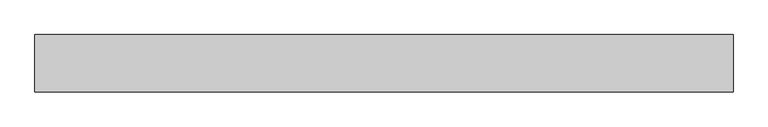
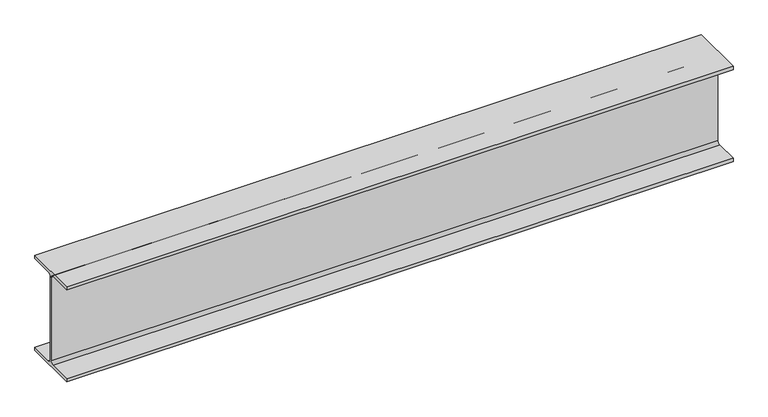
"""IFC4 building model written with IfcOpenShell, lengths in millimetres: beam geometry, Old_Steel Beam_H-KSD3502 : H_SB_ASB_H-194×150x6x9."""

from ifc_helpers import new_model, si_unit, point, frame, frame_2d, origin, place, context, project, spatial, polyline, circle_curve, trimmed, segment, composite_curve, outline, extrude, source, transform, mapped, element, save


def beam_e603d65a(model_context):
    return source(origin(), model_context, "Body", "SweptSolid", [
        extrude(outline(composite_curve([segment(polyline([(-82.5, -141.5), (-11.9, -141.5)]), True, "CONTINUOUS"), segment(trimmed(circle_curve(frame_2d((-11.9, -132.6)), 8.9), [point((-11.9, -141.5))], [point((-3.0, -132.6))], True, "CARTESIAN"), True, "CONTINUOUS"), segment(polyline([(-3.0, -132.6), (-3.0, 132.6)]), True, "CONTINUOUS"), segment(trimmed(circle_curve(frame_2d((-11.9, 132.6)), 8.9), [point((-3.0, 132.6))], [point((-11.9, 141.5))], True, "CARTESIAN"), True, "CONTINUOUS"), segment(polyline([(-11.9, 141.5), (-82.5, 141.5), (-82.5, 151.7), (82.5, 151.7), (82.5, 141.5), (11.9, 141.5)]), True, "CONTINUOUS"), segment(trimmed(circle_curve(frame_2d((11.9, 132.6)), 8.9), [point((11.9, 141.5))], [point((3.0, 132.6))], True, "CARTESIAN"), True, "CONTINUOUS"), segment(polyline([(3.0, 132.6), (3.0, -132.6)]), True, "CONTINUOUS"), segment(trimmed(circle_curve(frame_2d((11.9, -132.6)), 8.9), [point((3.0, -132.6))], [point((11.9, -141.5))], True, "CARTESIAN"), True, "CONTINUOUS"), segment(polyline([(11.9, -141.5), (82.5, -141.5), (82.5, -151.7), (-82.5, -151.7), (-82.5, -141.5)]), True, "CONTINUOUS")], self_intersect=False)), frame((-1171.2564634, 0.0, 0.0), z_axis=(1.0, 0.0, 0.0), x_axis=(0.0, 1.0, 0.0)), (0.0, 0.0, 1.0), 2006.3303739),
    ])


if __name__ == "__main__":
    model = new_model("IFC4")
    model_context = context("Model", 3, world=origin())
    ifc_project = project(units=[si_unit("LENGTHUNIT", "METRE", prefix="MILLI")], contexts=[model_context])
    site = spatial("IfcSite", under=ifc_project)
    building = spatial("IfcBuilding", under=site)
    placement = place(None, origin())
    beam_shape = beam_e603d65a(model_context)
    element("IfcBeam", 1, ObjectType="Old_Steel Beam_H-KSD3502 : H_SB_ASB_H-194×150x6x9", at=placement, inside=building, context=model_context, shape_type="MappedRepresentation", body=[
        mapped(beam_shape, transform((0.0, 0.0, 0.0), x_axis=(1.0, 0.0, 0.0), y_axis=(0.0, 1.0, 0.0), z_axis=(0.0, 0.0, 1.0))),
    ])
    save(model, "model.ifc")

# Revit data of these elements
# Type "Old_Steel Beam_H-KSD3502 : H_SB_ASB_H-194×150x6x9"
#   Width = 15.0 cm
#   Web Thickness = 0.6 cm
#   Web Fillet = 1.3 cm
#   Warping Constant = 43316.0 cm⁶
#   Torsional Moment of Inertia = 8.622 cm⁴
#   Torsional Modulus = 1.0 cm³
#   Section Area = 39.01 cm²
#   Plastic Modulus weak axis = 104.0 cm³
#   Plastic Modulus strong axis = 309.0 cm³
#   Perimeter = 0.95 m²/m
#   Nominal Weight = 30.60 kgf/m
#   Moment of Inertia weak axis = 507.00 cm⁴
#   Moment of Inertia strong axis = 2690.00 cm⁴
#   Height = 19.4 cm
#   Flange Thickness = 0.9 cm
#   Elastic Modulus weak axis = 67.6 cm³
#   Elastic Modulus strong axis = 277.0 cm³
#   Centroid Vertical = 9.7 cm
#   Centroid Horizontal = 7.5 cm
#   Length [instance default] = 1.5240 m
#   Structural Material [instance default] = Steel, 45-345
#   Assembly Code = ""
# Element 1 (IfcBeam, "Old_Steel Beam_H-KSD3502 : H_SB_ASB_H-194×150x6x9")
#   Structural Material = none
# Materials
#   "Steel, 45-345": class "Metal", colour RGB 189 187 185, transparency 0, Description = "Steel 345 MPa", Cost = 0
